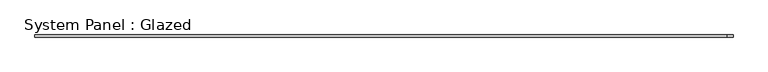
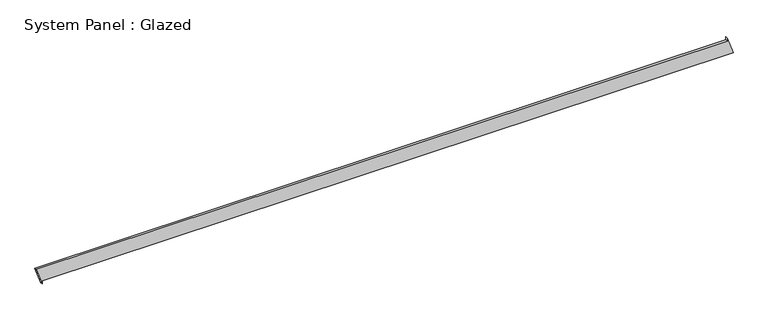
"""IFC4 building model written with IfcOpenShell, lengths in millimetres: plate geometry, System Panel : Glazed."""

import ifcopenshell
import ifcopenshell.guid

model = None  # the IFC model being written
_history = None  # IfcOwnerHistory: only IFC2X3 demands one
_inside = {}  # id of a spatial element -> (the spatial element, [elements in it])
_under = {}  # id of a project, library or spatial element -> (it, [spatial elements below it])
_declared = {}  # id of a project -> (the project, [libraries it declares])
_typed = {}  # id of a type object -> (the type object, [elements of that type])
_made_of = {}  # id of a material, layer set ... -> (it, [elements and type objects made of it])


def new_model(schema):
    """Start an empty IFC model of exactly this schema.

    Asked for "IFC4X3", IfcOpenShell would pick the latest addendum, in which some entities
    have other attributes; the version numbers below select the first issue.
    IFC2X3 requires an IfcOwnerHistory on every rooted entity: one is made here for all.
    """
    global model, _history
    if schema == "IFC4X3":
        model = ifcopenshell.file(schema_version=(4, 3, 0, 0))
    else:
        model = ifcopenshell.file(schema=schema)
    _inside.clear()
    _under.clear()
    _declared.clear()
    _typed.clear()
    _made_of.clear()
    _history = None
    if model.schema == "IFC2X3":
        org = make("IfcOrganization", Name="unknown")
        user = make(
            "IfcPersonAndOrganization",
            ThePerson=make("IfcPerson", FamilyName="unknown"),
            TheOrganization=org,
        )
        app = make(
            "IfcApplication",
            ApplicationDeveloper=org,
            Version="unknown",
            ApplicationFullName="unknown",
            ApplicationIdentifier="unknown",
        )
        _history = make(
            "IfcOwnerHistory",
            OwningUser=user,
            OwningApplication=app,
            ChangeAction="ADDED",
            CreationDate=0,
        )
    return model


def make(cls, **values):
    """One entity of the class cls with the attributes given. An attribute that is None is left unset."""
    return model.create_entity(
        cls, **{name: value for name, value in values.items() if value is not None}
    )


def rooted(cls, **values):
    """An entity with a GlobalId (a new one), such as an element, a storey or a relation."""
    return make(cls, GlobalId=ifcopenshell.guid.new(), OwnerHistory=_history, **values)


def si_unit(unit_type, name, prefix=None):
    """IfcSIUnit, for example si_unit("LENGTHUNIT", "METRE", prefix="MILLI")."""
    return make("IfcSIUnit", UnitType=unit_type, Prefix=prefix, Name=name)


def assignment(units):
    """IfcUnitAssignment: the units of a project."""
    return None if units is None else make("IfcUnitAssignment", Units=units)


def point(xyz):
    """IfcCartesianPoint."""
    return None if xyz is None else make("IfcCartesianPoint", Coordinates=xyz)


def direction(xyz):
    """IfcDirection."""
    return None if xyz is None else make("IfcDirection", DirectionRatios=xyz)


def frame(location, z_axis=None, x_axis=None):
    """IfcAxis2Placement3D, a coordinate frame: its origin and axes. An axis left out is left unset."""
    return make(
        "IfcAxis2Placement3D",
        Location=point(location),
        Axis=direction(z_axis),
        RefDirection=direction(x_axis),
    )


def origin():
    """The frame at (0, 0, 0) with its axes left unset."""
    return frame((0.0, 0.0, 0.0))


def place(relative_to, where):
    """IfcLocalPlacement: puts the frame where relative to a parent placement (None: the world)."""
    return make(
        "IfcLocalPlacement", PlacementRelTo=relative_to, RelativePlacement=where
    )


def context(
    kind, dimensions, precision=None, world=None, true_north=None, identifier=None
):
    """IfcGeometricRepresentationContext, for example the 3D "Model" context."""
    return make(
        "IfcGeometricRepresentationContext",
        ContextIdentifier=identifier,
        ContextType=kind,
        CoordinateSpaceDimension=dimensions,
        Precision=precision,
        WorldCoordinateSystem=world,
        TrueNorth=true_north,
    )


def project(units=None, contexts=None):
    """IfcProject with its units and contexts."""
    return rooted(
        "IfcProject",
        Name="project",
        RepresentationContexts=contexts,
        UnitsInContext=assignment(units),
    )


def spatial(cls, under=None, at=None, **own):
    """A site, building, storey or space (cls), placed at a placement, below another one or the project."""
    s = rooted(cls, ObjectPlacement=at, **own)
    if under is not None:
        _under.setdefault(under.id(), (under, []))[1].append(s)
    return s


def polyline(points):
    """IfcPolyline through the points."""
    return make("IfcPolyline", Points=[point(p) for p in points])


def outline(outer, holes=None, kind="AREA"):
    """IfcArbitraryClosedProfileDef: a profile drawn as a closed curve; with holes, ...WithVoids."""
    if holes is None:
        return make("IfcArbitraryClosedProfileDef", ProfileType=kind, OuterCurve=outer)
    return make(
        "IfcArbitraryProfileDefWithVoids",
        ProfileType=kind,
        OuterCurve=outer,
        InnerCurves=holes,
    )


def extrude(swept, where, along, depth):
    """IfcExtrudedAreaSolid: the profile swept, set in the frame where, extruded along a direction by depth."""
    return make(
        "IfcExtrudedAreaSolid",
        SweptArea=swept,
        Position=where,
        ExtrudedDirection=direction(along),
        Depth=depth,
    )


def shape(context_of_items, identifier, shape_type, items):
    """IfcShapeRepresentation: the items that make up one representation, for example the "Body"."""
    return make(
        "IfcShapeRepresentation",
        ContextOfItems=context_of_items,
        RepresentationIdentifier=identifier,
        RepresentationType=shape_type,
        Items=items,
    )


def source(mapping_origin, context_of_items, identifier, shape_type, items):
    """IfcRepresentationMap: a shape defined once, which mapped items show again and again."""
    return make(
        "IfcRepresentationMap",
        MappingOrigin=mapping_origin,
        MappedRepresentation=shape(context_of_items, identifier, shape_type, items),
    )


def transform(
    local_origin,
    x_axis=None,
    y_axis=None,
    z_axis=None,
    scale=None,
    scale2=None,
    scale3=None,
    uniform=True,
):
    """IfcCartesianTransformationOperator3D, or its non-uniform kind. x_axis, y_axis, z_axis: its Axis1, 2, 3."""
    if uniform:
        return make(
            "IfcCartesianTransformationOperator3D",
            Axis1=direction(x_axis),
            Axis2=direction(y_axis),
            LocalOrigin=point(local_origin),
            Scale=scale,
            Axis3=direction(z_axis),
        )
    return make(
        "IfcCartesianTransformationOperator3DnonUniform",
        Axis1=direction(x_axis),
        Axis2=direction(y_axis),
        LocalOrigin=point(local_origin),
        Scale=scale,
        Axis3=direction(z_axis),
        Scale2=scale2,
        Scale3=scale3,
    )


def mapped(mapping_source, mapping_target):
    """IfcMappedItem: shows the shape of a source again, moved by a transform."""
    return make(
        "IfcMappedItem", MappingSource=mapping_source, MappingTarget=mapping_target
    )


def made_of(thing, what):
    """Note that an element or type object is made of a material, layer set ...; save() writes the relation."""
    if what is not None:
        _made_of.setdefault(what.id(), (what, []))[1].append(thing)
    return thing


def element(
    cls,
    number,
    at=None,
    inside=None,
    cuts=None,
    type_object=None,
    material=None,
    context=None,
    identifier="Body",
    shape_type=None,
    held_by="IfcProductDefinitionShape",
    body=None,
    shapes=None,
    **own,
):
    """One element of the class cls, such as IfcWall. Its Tag is "e" and its number.

    at: its placement. inside: the storey or other place that contains it. cuts: it is an
    opening in that element (IfcRelVoidsElement). A single representation is given by context,
    identifier, shape_type and body (its items); several are given by shapes. held_by: the class
    of the entity that holds the representations. save() writes the other relations.
    """
    e = rooted(cls, Tag="e%d" % number, ObjectPlacement=at, **own)
    if body is not None:
        shapes = [shape(context, identifier, shape_type, body)]
    if shapes is not None:
        e.Representation = make(held_by, Representations=shapes)
    if inside is not None:
        _inside.setdefault(inside.id(), (inside, []))[1].append(e)
    if cuts is not None:
        rooted(
            "IfcRelVoidsElement", RelatingBuildingElement=cuts, RelatedOpeningElement=e
        )
    if type_object is not None:
        _typed.setdefault(type_object.id(), (type_object, []))[1].append(e)
    return made_of(e, material)


def aggregate(whole, parts):
    """IfcRelAggregates: a whole, such as a stair, and the parts it consists of."""
    return rooted("IfcRelAggregates", RelatingObject=whole, RelatedObjects=parts)


def save(model, path):
    """Write the relations noted so far, then the file.

    IfcRelAggregates (storeys below a building ...), IfcRelContainedInSpatialStructure (elements
    in a storey), IfcRelDefinesByType, IfcRelAssociatesMaterial and IfcRelDeclares: one each for
    every whole, place, type object, material and project.
    """
    for whole, parts in _under.values():
        aggregate(whole, parts)
    for where, things in _inside.values():
        rooted(
            "IfcRelContainedInSpatialStructure",
            RelatedElements=things,
            RelatingStructure=where,
        )
    for kind, things in _typed.values():
        rooted("IfcRelDefinesByType", RelatedObjects=things, RelatingType=kind)
    for what, things in _made_of.values():
        rooted("IfcRelAssociatesMaterial", RelatedObjects=things, RelatingMaterial=what)
    for by, libraries in _declared.values():
        rooted("IfcRelDeclares", RelatingContext=by, RelatedDefinitions=libraries)
    model.write(path)


def system_panel_glazed_13b512fd(model_context):
    return source(origin(), model_context, "Body", "SweptSolid", [
        extrude(outline(polyline([(0.0, -3959.20642), (35.3553391, -3959.20642), (35.3553391, 4028.228324), (235.5969396, 3959.1733726), (200.2416005, 3959.173312), (200.2552692, -4028.228324), (0.0, -3959.20642)])), frame((0.0, -49.5, 0.0), z_axis=(0.0, 1.0, 0.0), x_axis=(0.0, 0.0, 1.0)), (0.0, 0.0, 1.0), 25.0),
    ])


if __name__ == "__main__":
    model = new_model("IFC4")
    model_context = context("Model", 3, world=origin())
    ifc_project = project(units=[si_unit("LENGTHUNIT", "METRE", prefix="MILLI")], contexts=[model_context])
    site = spatial("IfcSite", under=ifc_project)
    building = spatial("IfcBuilding", under=site)
    placement = place(None, origin())
    system_panel_glazed_shape = system_panel_glazed_13b512fd(model_context)
    element("IfcPlate", 1, ObjectType="System Panel : Glazed", at=placement, inside=building, context=model_context, shape_type="MappedRepresentation", body=[
        mapped(system_panel_glazed_shape, transform((0.0, 0.0, 0.0), x_axis=(1.0, 0.0, 0.0), y_axis=(0.0, 1.0, 0.0), z_axis=(0.0, 0.0, 1.0))),
    ])
    save(model, "model.ifc")

# Revit data of these elements
# Element 1 (IfcPlate, "System Panel : Glazed")
#   Materials on its faces: "Glass"
# Materials
#   "Glass": class "Glass", colour RGB 218 227 224, transparency 0.85, Description = "Soda Lime Glass", Cost = 0
